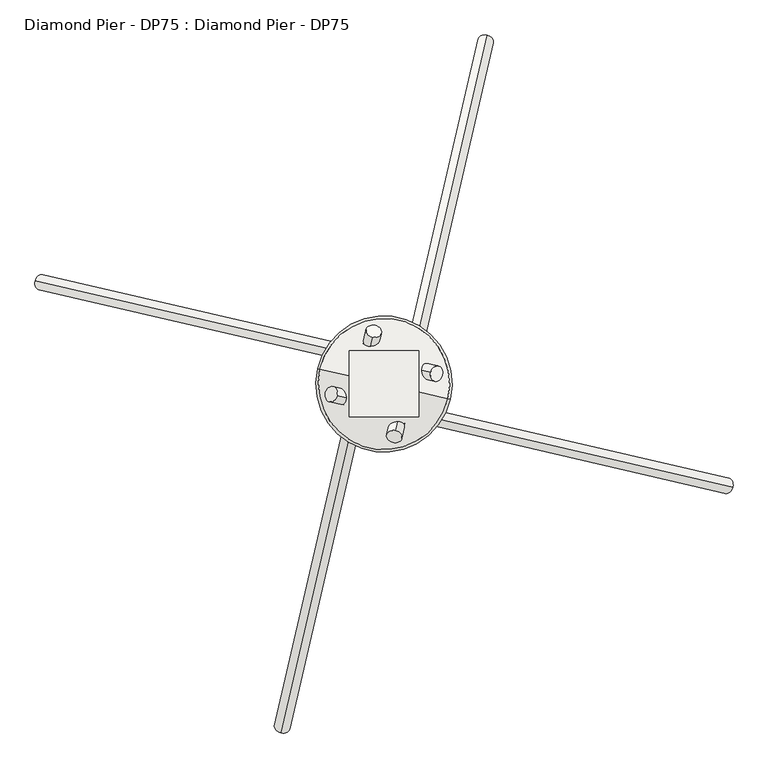
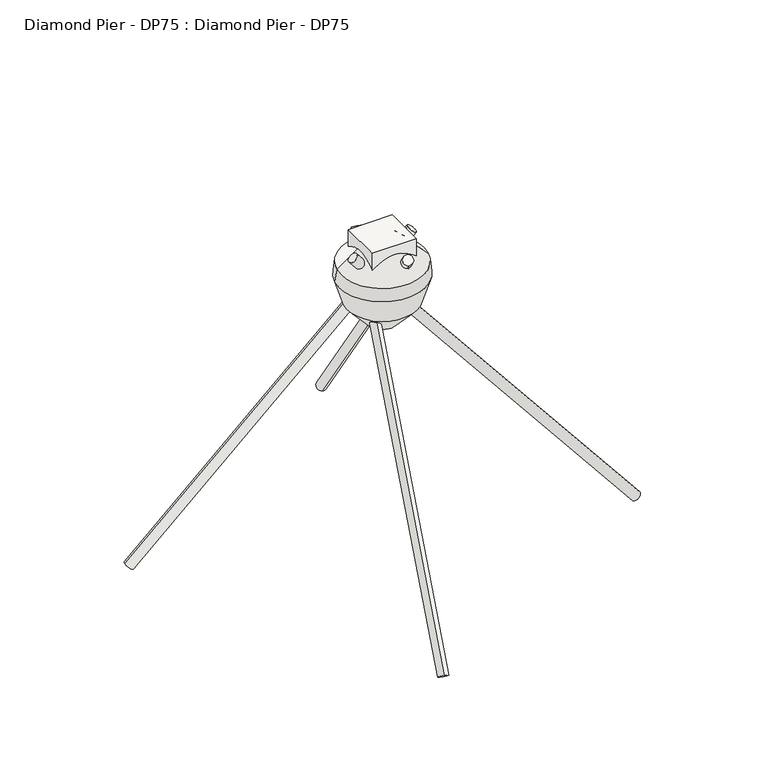
"""IFC4 building model written with IfcOpenShell, lengths in millimetres: slab geometry, Diamond Pier - DP75 : Diamond Pier - DP75."""

from ifc_helpers import new_model, si_unit, point, frame, frame_2d, origin, place, context, project, spatial, polyline, circle_curve, trimmed, segment, composite_curve, outline, extrude, source, transform, mapped, element, save
from ifc_brep_helpers import plane_surface, revolved_surface, advanced_brep


def diamond_pier_dp75_diamond_pier_dp75_ae65de88(model_context):
    return source(origin(), model_context, "Body", "SolidModel", [
        extrude(outline(composite_curve([segment(trimmed(circle_curve(frame_2d((1e-07, -15.875)), 15.875), [point((1e-07, -31.7500001))], [point((0.0, 0.0))], False, "CARTESIAN"), True, "CONTINUOUS"), segment(trimmed(circle_curve(frame_2d((1e-07, -15.875)), 15.875), [point((0.0, 0.0))], [point((1e-07, -31.7500001))], False, "CARTESIAN"), True, "CONTINUOUS")], self_intersect=False)), frame((-207.7929333, -703.2724242, -991.3584593), z_axis=(0.14520854647133766, 0.628002114484006, 0.7645441924671841), x_axis=(-0.9742942350214497, 0.2252792569322976, 0.0)), (0.0, 0.0, 1.0), 1270.0),
        extrude(outline(composite_curve([segment(trimmed(circle_curve(frame_2d((1e-07, -15.875)), 15.875), [point((1e-07, -31.7500001))], [point((0.0, 0.0))], False, "CARTESIAN"), True, "CONTINUOUS"), segment(trimmed(circle_curve(frame_2d((1e-07, -15.875)), 15.875), [point((0.0, 0.0))], [point((1e-07, -31.7500001))], False, "CARTESIAN"), True, "CONTINUOUS")], self_intersect=False)), frame((-703.2724242, 207.7929333, -991.3584593), z_axis=(0.6280021144840067, -0.14520854647133485, 0.7645441924671843), x_axis=(0.22527925693229323, 0.9742942350214507, 0.0)), (0.0, 0.0, 1.0), 1270.0),
        extrude(outline(composite_curve([segment(trimmed(circle_curve(frame_2d((1e-07, -15.875)), 15.875), [point((1e-07, -31.7500001))], [point((0.0, 0.0))], False, "CARTESIAN"), True, "CONTINUOUS"), segment(trimmed(circle_curve(frame_2d((1e-07, -15.875)), 15.875), [point((0.0, 0.0))], [point((1e-07, -31.7500001))], False, "CARTESIAN"), True, "CONTINUOUS")], self_intersect=False)), frame((207.7929333, 703.2724242, -991.3584593), z_axis=(-0.14520854647133596, -0.6280021144840063, 0.7645441924671844), x_axis=(0.9742942350214504, -0.22527925693229495, 0.0)), (0.0, 0.0, 1.0), 1270.0),
        extrude(outline(composite_curve([segment(trimmed(circle_curve(frame_2d((1e-07, -15.875)), 15.875), [point((1e-07, -31.7500001))], [point((0.0, 0.0))], False, "CARTESIAN"), True, "CONTINUOUS"), segment(trimmed(circle_curve(frame_2d((1e-07, -15.875)), 15.875), [point((0.0, 0.0))], [point((1e-07, -31.7500001))], False, "CARTESIAN"), True, "CONTINUOUS")], self_intersect=False)), frame((703.2724242, -207.7929333, -991.3584593), z_axis=(-0.6280021144840057, 0.14520854647133877, 0.7645441924671843), x_axis=(-0.22527925693229922, -0.9742942350214493, 0.0)), (0.0, 0.0, 1.0), 1270.0),
        advanced_brep(
        [(-108.3324504, 25.0489565, -217.3055075), (108.3324504, -25.0489565, -217.3055075), (42.5837569, -9.8463449, -291.7305661), (-42.5837569, 9.8463449, -291.7305661), (-133.8544614, 30.950233, -132.1736467), (133.8544614, -30.950233, -132.1736467), (-128.9734508, 29.821631, -90.9283538), (128.9734508, -29.821631, -90.9283538), (-48.2749795, 11.1622866, -12.7), (48.2749795, -11.1622866, -12.7), (0.0, 0.0, -12.7), (0.0, 0.0, -292.024192)],
        [
            (0, 1, circle_curve(frame((0.0, 0.0, -217.3055075), z_axis=(0.0, 0.0, -1.0), x_axis=(0.9742942350214493, -0.22527925693229933, 0.0)), 111.1906922)),
            (1, 2),
            (2, 3, circle_curve(frame((0.0, 0.0, -291.7305661), z_axis=(0.0, 0.0, 1.0), x_axis=(0.9742942350214493, -0.22527925693229933, 0.0)), 43.7072861)),
            (3, 0),
            (1, 0, circle_curve(frame((0.0, 0.0, -217.3055075), z_axis=(0.0, 0.0, -1.0), x_axis=(0.9742942350214493, -0.22527925693229933, 0.0)), 111.1906922)),
            (3, 2, circle_curve(frame((0.0, 0.0, -291.7305661), z_axis=(0.0, 0.0, 1.0), x_axis=(0.9742942350214493, -0.22527925693229933, 0.0)), 43.7072861)),
            (4, 5, circle_curve(frame((0.0, 0.0, -132.1736467), z_axis=(0.0, 0.0, -1.0), x_axis=(0.9742942350214493, -0.22527925693229933, 0.0)), 137.3860755)),
            (5, 1),
            (0, 4),
            (5, 4, circle_curve(frame((0.0, 0.0, -132.1736467), z_axis=(0.0, 0.0, -1.0), x_axis=(0.9742942350214493, -0.22527925693229933, 0.0)), 137.3860755)),
            (6, 7, circle_curve(frame((0.0, 0.0, -90.9283538), z_axis=(0.0, 0.0, -1.0), x_axis=(0.9742942350214493, -0.22527925693229933, 0.0)), 132.3762845)),
            (7, 5),
            (4, 6),
            (7, 6, circle_curve(frame((0.0, 0.0, -90.9283538), z_axis=(0.0, 0.0, -1.0), x_axis=(0.9742942350214493, -0.22527925693229933, 0.0)), 132.3762845)),
            (8, 9, circle_curve(frame((0.0, 0.0, -12.7), z_axis=(0.0, 0.0, -1.0), x_axis=(0.9742942350214493, -0.22527925693229933, 0.0)), 49.5486659)),
            (9, 7),
            (6, 8),
            (9, 8, circle_curve(frame((0.0, 0.0, -12.7), z_axis=(0.0, 0.0, -1.0), x_axis=(0.9742942350214493, -0.22527925693229933, 0.0)), 49.5486659)),
            (10, 9),
            (8, 10),
            (2, 11),
            (11, 3),
        ],
        [
            revolved_surface(polyline([(42.5837569, -9.8463449, -291.7305661), (108.3324504, -25.0489565, -217.3055075)]), (0.0, 0.0, -12.7), (0.0, 0.0, 1.0)),
            revolved_surface(polyline([(108.3324504, -25.0489565, -217.3055075), (133.8544614, -30.950233, -132.1736467)]), (0.0, 0.0, -12.7), (0.0, 0.0, 1.0)),
            revolved_surface(polyline([(133.8544614, -30.950233, -132.1736467), (128.9734508, -29.821631, -90.9283538)]), (0.0, 0.0, -12.7), (0.0, 0.0, 1.0)),
            revolved_surface(polyline([(128.9734508, -29.821631, -90.9283538), (48.2749795, -11.1622866, -12.7)]), (0.0, 0.0, -12.7), (0.0, 0.0, 1.0)),
            plane_surface(frame((0.0, 0.0, -12.7), z_axis=(0.0, 0.0, 1.0), x_axis=(0.9742942350214493, -0.22527925693229933, 0.0))),
            revolved_surface(polyline([(0.0, 0.0, -292.024192), (42.5837569, -9.8463449, -291.7305661)]), (0.0, 0.0, -12.7), (0.0, 0.0, 1.0)),
        ],
        [
            (0, [[1, 2, 3, 4]]),
            (0, [[5, -4, 6, -2]]),
            (1, [[7, 8, -1, 9]]),
            (1, [[10, -9, -5, -8]]),
            (2, [[11, 12, -7, 13]]),
            (2, [[14, -13, -10, -12]]),
            (3, [[15, 16, -11, 17]]),
            (3, [[18, -17, -14, -16]]),
            (4, [[19, -15, 20]]),
            (4, [[-20, -18, -19]]),
            (5, [[-3, 21, 22]]),
            (5, [[-6, -22, -21]]),
        ],
    ),
        extrude(outline(polyline([(70.369164, 66.5326915), (70.369164, -66.5326915), (-70.369164, -66.5326915), (-70.369164, 66.5326915), (70.369164, 66.5326915)])), frame((0.0, 0.0, -87.3372243), z_axis=(0.0, 0.0, 1.0), x_axis=(1.0, 0.0, 0.0)), (0.0, 0.0, 1.0), 87.3372243),
    ])


if __name__ == "__main__":
    model = new_model("IFC4")
    model_context = context("Model", 3, world=origin())
    ifc_project = project(units=[si_unit("LENGTHUNIT", "METRE", prefix="MILLI")], contexts=[model_context])
    site = spatial("IfcSite", under=ifc_project)
    building = spatial("IfcBuilding", under=site)
    placement = place(None, origin())
    diamond_pier_dp75_diamond_pier_dp75_shape = diamond_pier_dp75_diamond_pier_dp75_ae65de88(model_context)
    element("IfcSlab", 1, ObjectType="Diamond Pier - DP75 : Diamond Pier - DP75", at=placement, inside=building, context=model_context, shape_type="MappedRepresentation", body=[
        mapped(diamond_pier_dp75_diamond_pier_dp75_shape, transform((0.0, 0.0, 0.0), x_axis=(1.0, 0.0, 0.0), y_axis=(0.0, 1.0, 0.0), z_axis=(0.0, 0.0, 1.0))),
    ])
    save(model, "model.ifc")

# Revit data of these elements
# Type "Diamond Pier - DP75 : Diamond Pier - DP75"
#   Assembly Code = "A1010100"
#   Structural Material = DIAMOND PIER DP-50/50 - (3300# B.L.C. AT 1500PSF SOILS, 4400# B.L.C. AT 2000PSF SOILS)
# Element 1 (IfcSlab, "Diamond Pier - DP75 : Diamond Pier - DP75")
#   Materials on its faces: "DIAMOND PIER DP-50/50 - (3300# B.L.C. AT 1500PSF SOILS, 4400# B.L.C. AT 2000PSF SOILS)"
# Materials
#   "DIAMOND PIER DP-50/50 - (3300# B.L.C. AT 1500PSF SOILS, 4400# B.L.C. AT 2000PSF SOILS)": class "Generic", colour RGB 195 195 195, transparency 0, Cost = 0
